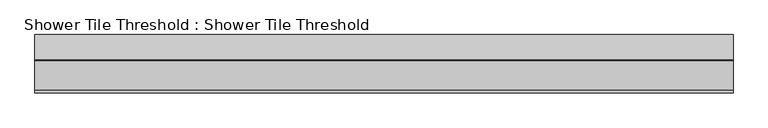
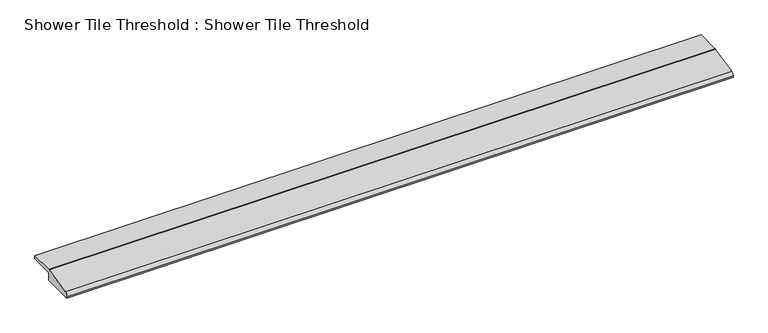
"""IFC4 building model written with IfcOpenShell, lengths in millimetres: proxy geometry, Shower Tile Threshold : Shower Tile Threshold."""

import ifcopenshell
import ifcopenshell.guid

model = None  # the IFC model being written
_history = None  # IfcOwnerHistory: only IFC2X3 demands one
_inside = {}  # id of a spatial element -> (the spatial element, [elements in it])
_under = {}  # id of a project, library or spatial element -> (it, [spatial elements below it])
_declared = {}  # id of a project -> (the project, [libraries it declares])
_typed = {}  # id of a type object -> (the type object, [elements of that type])
_made_of = {}  # id of a material, layer set ... -> (it, [elements and type objects made of it])


def new_model(schema):
    """Start an empty IFC model of exactly this schema.

    Asked for "IFC4X3", IfcOpenShell would pick the latest addendum, in which some entities
    have other attributes; the version numbers below select the first issue.
    IFC2X3 requires an IfcOwnerHistory on every rooted entity: one is made here for all.
    """
    global model, _history
    if schema == "IFC4X3":
        model = ifcopenshell.file(schema_version=(4, 3, 0, 0))
    else:
        model = ifcopenshell.file(schema=schema)
    _inside.clear()
    _under.clear()
    _declared.clear()
    _typed.clear()
    _made_of.clear()
    _history = None
    if model.schema == "IFC2X3":
        org = make("IfcOrganization", Name="unknown")
        user = make(
            "IfcPersonAndOrganization",
            ThePerson=make("IfcPerson", FamilyName="unknown"),
            TheOrganization=org,
        )
        app = make(
            "IfcApplication",
            ApplicationDeveloper=org,
            Version="unknown",
            ApplicationFullName="unknown",
            ApplicationIdentifier="unknown",
        )
        _history = make(
            "IfcOwnerHistory",
            OwningUser=user,
            OwningApplication=app,
            ChangeAction="ADDED",
            CreationDate=0,
        )
    return model


def make(cls, **values):
    """One entity of the class cls with the attributes given. An attribute that is None is left unset."""
    return model.create_entity(
        cls, **{name: value for name, value in values.items() if value is not None}
    )


def rooted(cls, **values):
    """An entity with a GlobalId (a new one), such as an element, a storey or a relation."""
    return make(cls, GlobalId=ifcopenshell.guid.new(), OwnerHistory=_history, **values)


def si_unit(unit_type, name, prefix=None):
    """IfcSIUnit, for example si_unit("LENGTHUNIT", "METRE", prefix="MILLI")."""
    return make("IfcSIUnit", UnitType=unit_type, Prefix=prefix, Name=name)


def assignment(units):
    """IfcUnitAssignment: the units of a project."""
    return None if units is None else make("IfcUnitAssignment", Units=units)


def point(xyz):
    """IfcCartesianPoint."""
    return None if xyz is None else make("IfcCartesianPoint", Coordinates=xyz)


def direction(xyz):
    """IfcDirection."""
    return None if xyz is None else make("IfcDirection", DirectionRatios=xyz)


def frame(location, z_axis=None, x_axis=None):
    """IfcAxis2Placement3D, a coordinate frame: its origin and axes. An axis left out is left unset."""
    return make(
        "IfcAxis2Placement3D",
        Location=point(location),
        Axis=direction(z_axis),
        RefDirection=direction(x_axis),
    )


def frame_2d(location, x_axis=None):
    """IfcAxis2Placement2D, a coordinate frame in the plane: its origin and x axis."""
    return make(
        "IfcAxis2Placement2D", Location=point(location), RefDirection=direction(x_axis)
    )


def origin():
    """The frame at (0, 0, 0) with its axes left unset."""
    return frame((0.0, 0.0, 0.0))


def place(relative_to, where):
    """IfcLocalPlacement: puts the frame where relative to a parent placement (None: the world)."""
    return make(
        "IfcLocalPlacement", PlacementRelTo=relative_to, RelativePlacement=where
    )


def context(
    kind, dimensions, precision=None, world=None, true_north=None, identifier=None
):
    """IfcGeometricRepresentationContext, for example the 3D "Model" context."""
    return make(
        "IfcGeometricRepresentationContext",
        ContextIdentifier=identifier,
        ContextType=kind,
        CoordinateSpaceDimension=dimensions,
        Precision=precision,
        WorldCoordinateSystem=world,
        TrueNorth=true_north,
    )


def project(units=None, contexts=None):
    """IfcProject with its units and contexts."""
    return rooted(
        "IfcProject",
        Name="project",
        RepresentationContexts=contexts,
        UnitsInContext=assignment(units),
    )


def spatial(cls, under=None, at=None, **own):
    """A site, building, storey or space (cls), placed at a placement, below another one or the project."""
    s = rooted(cls, ObjectPlacement=at, **own)
    if under is not None:
        _under.setdefault(under.id(), (under, []))[1].append(s)
    return s


def polyline(points):
    """IfcPolyline through the points."""
    return make("IfcPolyline", Points=[point(p) for p in points])


def circle_curve(where, radius):
    """IfcCircle in the frame where."""
    return make("IfcCircle", Position=where, Radius=radius)


def trimmed(basis, trim1, trim2, sense, master):
    """IfcTrimmedCurve: the piece of a basis curve between two trims."""
    return make(
        "IfcTrimmedCurve",
        BasisCurve=basis,
        Trim1=trim1,
        Trim2=trim2,
        SenseAgreement=sense,
        MasterRepresentation=master,
    )


def segment(curve, same_sense, transition):
    """IfcCompositeCurveSegment."""
    return make(
        "IfcCompositeCurveSegment",
        Transition=transition,
        SameSense=same_sense,
        ParentCurve=curve,
    )


def composite_curve(segments, self_intersect=None):
    """IfcCompositeCurve: segments joined end to end."""
    return make("IfcCompositeCurve", Segments=segments, SelfIntersect=self_intersect)


def outline(outer, holes=None, kind="AREA"):
    """IfcArbitraryClosedProfileDef: a profile drawn as a closed curve; with holes, ...WithVoids."""
    if holes is None:
        return make("IfcArbitraryClosedProfileDef", ProfileType=kind, OuterCurve=outer)
    return make(
        "IfcArbitraryProfileDefWithVoids",
        ProfileType=kind,
        OuterCurve=outer,
        InnerCurves=holes,
    )


def extrude(swept, where, along, depth):
    """IfcExtrudedAreaSolid: the profile swept, set in the frame where, extruded along a direction by depth."""
    return make(
        "IfcExtrudedAreaSolid",
        SweptArea=swept,
        Position=where,
        ExtrudedDirection=direction(along),
        Depth=depth,
    )


def shape(context_of_items, identifier, shape_type, items):
    """IfcShapeRepresentation: the items that make up one representation, for example the "Body"."""
    return make(
        "IfcShapeRepresentation",
        ContextOfItems=context_of_items,
        RepresentationIdentifier=identifier,
        RepresentationType=shape_type,
        Items=items,
    )


def source(mapping_origin, context_of_items, identifier, shape_type, items):
    """IfcRepresentationMap: a shape defined once, which mapped items show again and again."""
    return make(
        "IfcRepresentationMap",
        MappingOrigin=mapping_origin,
        MappedRepresentation=shape(context_of_items, identifier, shape_type, items),
    )


def transform(
    local_origin,
    x_axis=None,
    y_axis=None,
    z_axis=None,
    scale=None,
    scale2=None,
    scale3=None,
    uniform=True,
):
    """IfcCartesianTransformationOperator3D, or its non-uniform kind. x_axis, y_axis, z_axis: its Axis1, 2, 3."""
    if uniform:
        return make(
            "IfcCartesianTransformationOperator3D",
            Axis1=direction(x_axis),
            Axis2=direction(y_axis),
            LocalOrigin=point(local_origin),
            Scale=scale,
            Axis3=direction(z_axis),
        )
    return make(
        "IfcCartesianTransformationOperator3DnonUniform",
        Axis1=direction(x_axis),
        Axis2=direction(y_axis),
        LocalOrigin=point(local_origin),
        Scale=scale,
        Axis3=direction(z_axis),
        Scale2=scale2,
        Scale3=scale3,
    )


def mapped(mapping_source, mapping_target):
    """IfcMappedItem: shows the shape of a source again, moved by a transform."""
    return make(
        "IfcMappedItem", MappingSource=mapping_source, MappingTarget=mapping_target
    )


def made_of(thing, what):
    """Note that an element or type object is made of a material, layer set ...; save() writes the relation."""
    if what is not None:
        _made_of.setdefault(what.id(), (what, []))[1].append(thing)
    return thing


def element(
    cls,
    number,
    at=None,
    inside=None,
    cuts=None,
    type_object=None,
    material=None,
    context=None,
    identifier="Body",
    shape_type=None,
    held_by="IfcProductDefinitionShape",
    body=None,
    shapes=None,
    **own,
):
    """One element of the class cls, such as IfcWall. Its Tag is "e" and its number.

    at: its placement. inside: the storey or other place that contains it. cuts: it is an
    opening in that element (IfcRelVoidsElement). A single representation is given by context,
    identifier, shape_type and body (its items); several are given by shapes. held_by: the class
    of the entity that holds the representations. save() writes the other relations.
    """
    e = rooted(cls, Tag="e%d" % number, ObjectPlacement=at, **own)
    if body is not None:
        shapes = [shape(context, identifier, shape_type, body)]
    if shapes is not None:
        e.Representation = make(held_by, Representations=shapes)
    if inside is not None:
        _inside.setdefault(inside.id(), (inside, []))[1].append(e)
    if cuts is not None:
        rooted(
            "IfcRelVoidsElement", RelatingBuildingElement=cuts, RelatedOpeningElement=e
        )
    if type_object is not None:
        _typed.setdefault(type_object.id(), (type_object, []))[1].append(e)
    return made_of(e, material)


def aggregate(whole, parts):
    """IfcRelAggregates: a whole, such as a stair, and the parts it consists of."""
    return rooted("IfcRelAggregates", RelatingObject=whole, RelatedObjects=parts)


def save(model, path):
    """Write the relations noted so far, then the file.

    IfcRelAggregates (storeys below a building ...), IfcRelContainedInSpatialStructure (elements
    in a storey), IfcRelDefinesByType, IfcRelAssociatesMaterial and IfcRelDeclares: one each for
    every whole, place, type object, material and project.
    """
    for whole, parts in _under.values():
        aggregate(whole, parts)
    for where, things in _inside.values():
        rooted(
            "IfcRelContainedInSpatialStructure",
            RelatedElements=things,
            RelatingStructure=where,
        )
    for kind, things in _typed.values():
        rooted("IfcRelDefinesByType", RelatedObjects=things, RelatingType=kind)
    for what, things in _made_of.values():
        rooted("IfcRelAssociatesMaterial", RelatedObjects=things, RelatingMaterial=what)
    for by, libraries in _declared.values():
        rooted("IfcRelDeclares", RelatingContext=by, RelatedDefinitions=libraries)
    model.write(path)


def shower_tile_threshold_shower_tile_threshold_c9caed11(model_context):
    return source(origin(), model_context, "Body", "SweptSolid", [
        extrude(outline(composite_curve([segment(polyline([(-95.25, -20.6375), (-152.4, -20.6375), (-152.4, -17.7937897)]), True, "CONTINUOUS"), segment(trimmed(circle_curve(frame_2d((-146.05, -17.7937897)), 6.35), [point((-152.4, -17.7937897))], [point((-147.4275084, -11.5950019))], False, "CARTESIAN"), True, "CONTINUOUS"), segment(polyline([(-147.4275084, -11.5950019), (-95.9304548, -0.1512122)]), True, "CONTINUOUS"), segment(trimmed(circle_curve(frame_2d((-94.5529463, -6.35)), 6.35), [point((-95.9304548, -0.1512122))], [point((-94.5529463, 0.0))], False, "CARTESIAN"), True, "CONTINUOUS"), segment(polyline([(-94.5529463, 0.0), (-50.8, 0.0), (-50.8, -6.35), (-95.25, -6.35), (-95.25, -20.6375)]), True, "CONTINUOUS")], self_intersect=False)), frame((-914.4, 0.0, 0.0), z_axis=(1.0, 0.0, 0.0), x_axis=(0.0, 1.0, 0.0)), (0.0, 0.0, 1.0), 1219.2),
    ])


if __name__ == "__main__":
    model = new_model("IFC4")
    model_context = context("Model", 3, world=origin())
    ifc_project = project(units=[si_unit("LENGTHUNIT", "METRE", prefix="MILLI")], contexts=[model_context])
    site = spatial("IfcSite", under=ifc_project)
    building = spatial("IfcBuilding", under=site)
    placement = place(None, origin())
    shower_tile_threshold_shower_tile_threshold_shape = shower_tile_threshold_shower_tile_threshold_c9caed11(model_context)
    element("IfcBuildingElementProxy", 1, Name="Shower Tile Threshold : Shower Tile Threshold", ObjectType="Shower Tile Threshold : Shower Tile Threshold", at=placement, inside=building, context=model_context, shape_type="MappedRepresentation", body=[
        mapped(shower_tile_threshold_shower_tile_threshold_shape, transform((0.0, 0.0, 0.0), x_axis=(1.0, 0.0, 0.0), y_axis=(0.0, 1.0, 0.0), z_axis=(0.0, 0.0, 1.0))),
    ])
    save(model, "model.ifc")

# Revit data of these elements
# Type "Shower Tile Threshold : Shower Tile Threshold"
#   Width [instance default] = 2' - 0"
#   Offset [instance default] = 0' - 1"
#   Material = Tile, Porcelain, 4in
# Element 1 (IfcBuildingElementProxy, "Shower Tile Threshold : Shower Tile Threshold")
#   Width = 4' - 0"
#   Offset = 0' - 0.53229"
# Materials
#   "Tile, Porcelain, 4in": class "Generic", colour RGB 255 255 255, transparency 0, Description = "Porcelain tile, 4\", white", Cost = 0
